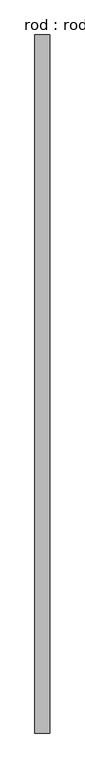
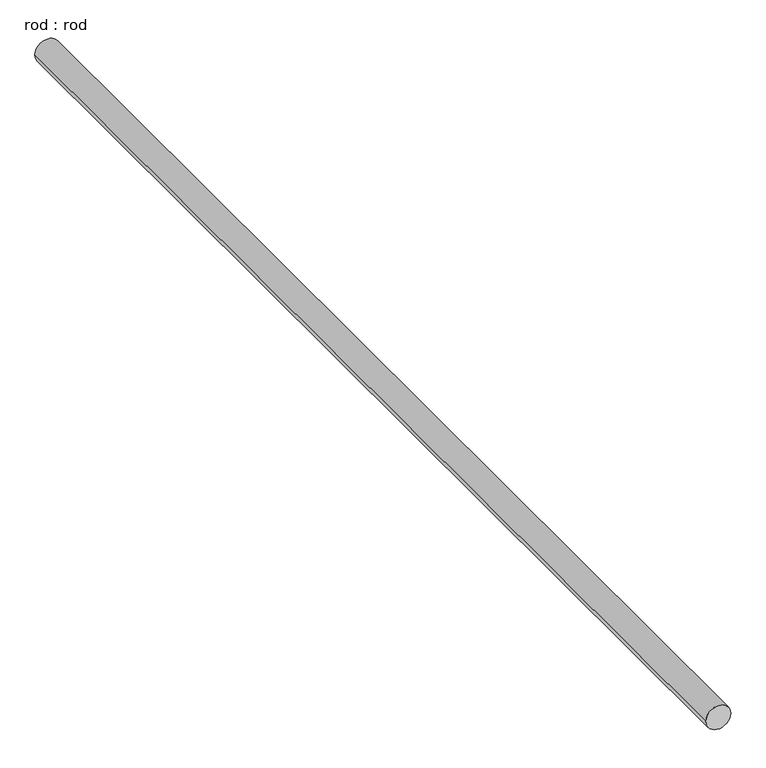
"""IFC4 building model written with IfcOpenShell, lengths in millimetres: proxy geometry, rod : rod."""

from ifc_helpers import new_model, si_unit, point, frame, frame_2d, origin, place, context, project, spatial, circle_curve, trimmed, segment, composite_curve, outline, extrude, source, transform, mapped, element, save


def rod_rod_61c26362(model_context):
    return source(origin(), model_context, "Body", "SweptSolid", [
        extrude(outline(composite_curve([segment(trimmed(circle_curve(frame_2d((0.0108462, 0.0)), 200.0), [point((0.0108462, 200.0))], [point((0.0108462, -200.0))], False, "CARTESIAN"), True, "CONTINUOUS"), segment(trimmed(circle_curve(frame_2d((0.0108462, 0.0)), 200.0), [point((0.0108462, -200.0))], [point((0.0108462, 200.0))], False, "CARTESIAN"), True, "CONTINUOUS")], self_intersect=False)), frame((0.0, -5298.4387775, 0.0), z_axis=(0.0, 1.0, 0.0), x_axis=(0.0, 0.0, 1.0)), (0.0, 0.0, 1.0), 18782.3347856),
    ])


if __name__ == "__main__":
    model = new_model("IFC4")
    model_context = context("Model", 3, world=origin())
    ifc_project = project(units=[si_unit("LENGTHUNIT", "METRE", prefix="MILLI")], contexts=[model_context])
    site = spatial("IfcSite", under=ifc_project)
    building = spatial("IfcBuilding", under=site)
    placement = place(None, origin())
    rod_rod_shape = rod_rod_61c26362(model_context)
    element("IfcBuildingElementProxy", 1, Name="rod : rod", ObjectType="rod : rod", at=placement, inside=building, context=model_context, shape_type="MappedRepresentation", body=[
        mapped(rod_rod_shape, transform((0.0, 0.0, 0.0), x_axis=(1.0, 0.0, 0.0), y_axis=(0.0, 1.0, 0.0), z_axis=(0.0, 0.0, 1.0))),
    ])
    save(model, "model.ifc")

# Revit data of these elements
# Type "rod : rod"
#   Default Elevation = 0
